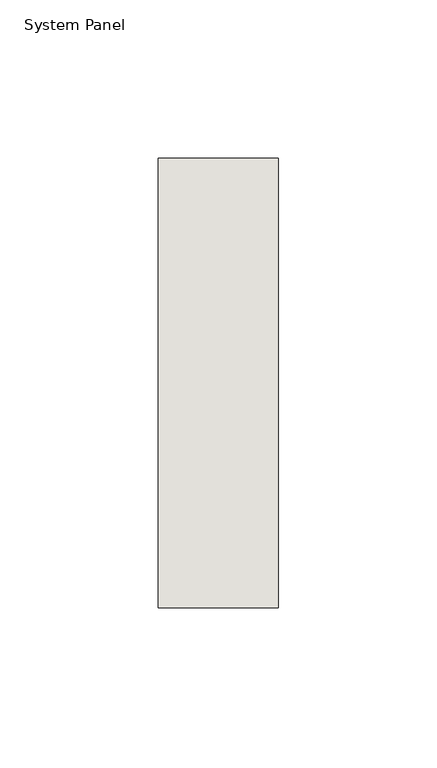
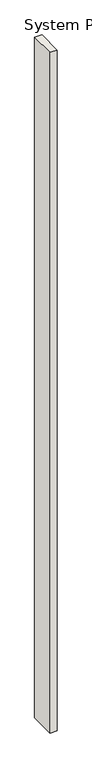
"""IFC4 building model written with IfcOpenShell, lengths in millimetres: wall geometry, System Panel : NLRS_21_CWP_hsb-vulling minerale wol 142 _gen_rsf."""

from ifc_helpers import new_model, si_unit, origin, origin_with_axes, place, context, project, spatial, polyline, outline, extrude, source, transform, mapped, element, save


def system_panel_13b21a00(model_context):
    return source(origin(), model_context, "Body", "SweptSolid", [
        extrude(outline(polyline([(18.9999998, -71.0), (-18.9999998, -71.0), (-18.9999998, 71.0), (18.9999998, 71.0), (18.9999998, -71.0)])), origin_with_axes(), (0.0, 0.0, 1.0), 3849.0),
    ])


if __name__ == "__main__":
    model = new_model("IFC4")
    model_context = context("Model", 3, world=origin())
    ifc_project = project(units=[si_unit("LENGTHUNIT", "METRE", prefix="MILLI")], contexts=[model_context])
    site = spatial("IfcSite", under=ifc_project)
    building = spatial("IfcBuilding", under=site)
    placement = place(None, origin())
    system_panel_shape = system_panel_13b21a00(model_context)
    element("IfcWall", 1, ObjectType="System Panel : NLRS_21_CWP_hsb-vulling minerale wol 142 _gen_rsf", at=placement, inside=building, context=model_context, shape_type="MappedRepresentation", body=[
        mapped(system_panel_shape, transform((0.0, 0.0, 0.0), x_axis=(1.0, 0.0, 0.0), y_axis=(0.0, 1.0, 0.0), z_axis=(0.0, 0.0, 1.0))),
    ])
    save(model, "model.ifc")

# Revit data of these elements
# Type "System Panel : NLRS_21_CWP_hsb-vulling minerale wol 142 _gen_rsf"
#   Type IfcGUID = "07M7mRoiH1CR8m_RSKIwpC"
#   Assembly Code = "21.23"
#   IfcExportAs = "IfcWall"
# Element 1 (IfcWall, "System Panel : NLRS_21_CWP_hsb-vulling minerale wol 142 _gen_rsf")
#   Materials on its faces: "NLRS_m1_isolatie minerale wol_gen_rsf"
# Materials
#   "NLRS_m1_isolatie minerale wol_gen_rsf": class "M - Anorganische materialen", colour RGB 200 200 140, transparency 0, Keynote = "m1", Manufacturer = "Revit Standards Foundation", URL = "www.revitstandards.org", Description = "isolatie minerale wol", Cost = 0
